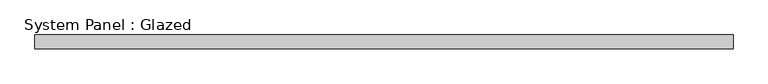
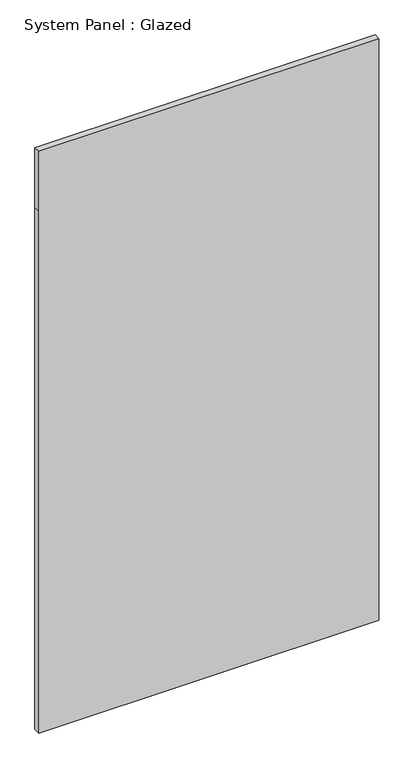
"""IFC4 building model written with IfcOpenShell, lengths in millimetres: plate geometry, System Panel : Glazed."""

from ifc_helpers import new_model, si_unit, frame, origin, place, context, project, spatial, polyline, outline, extrude, source, transform, mapped, element, save


def system_panel_glazed_c092dd15(model_context):
    return source(origin(), model_context, "Body", "SweptSolid", [
        extrude(outline(polyline([(0.0, -648.1535714), (0.0, 648.1535714), (2101.85, 648.1535714), (2343.15, 648.1535714), (2343.15, -648.1535714), (2101.85, -648.1535714), (0.0, -648.1535714)])), frame((0.0, 19.05, 0.0), z_axis=(0.0, 1.0, 0.0), x_axis=(0.0, 0.0, 1.0)), (0.0, 0.0, 1.0), 25.4),
    ])


if __name__ == "__main__":
    model = new_model("IFC4")
    model_context = context("Model", 3, world=origin())
    ifc_project = project(units=[si_unit("LENGTHUNIT", "METRE", prefix="MILLI")], contexts=[model_context])
    site = spatial("IfcSite", under=ifc_project)
    building = spatial("IfcBuilding", under=site)
    placement = place(None, origin())
    system_panel_glazed_shape = system_panel_glazed_c092dd15(model_context)
    element("IfcPlate", 1, ObjectType="System Panel : Glazed", at=placement, inside=building, context=model_context, shape_type="MappedRepresentation", body=[
        mapped(system_panel_glazed_shape, transform((0.0, 0.0, 0.0), x_axis=(1.0, 0.0, 0.0), y_axis=(0.0, 1.0, 0.0), z_axis=(0.0, 0.0, 1.0))),
    ])
    save(model, "model.ifc")

# Revit data of these elements
# Element 1 (IfcPlate, "System Panel : Glazed")
#   Materials on its faces: "Glass"
# Materials
#   "Glass": class "Glass", colour RGB 0 128 192, transparency 0.75, Cost = 0
